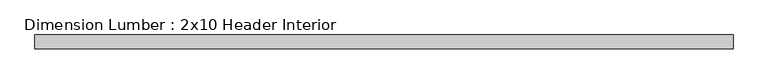
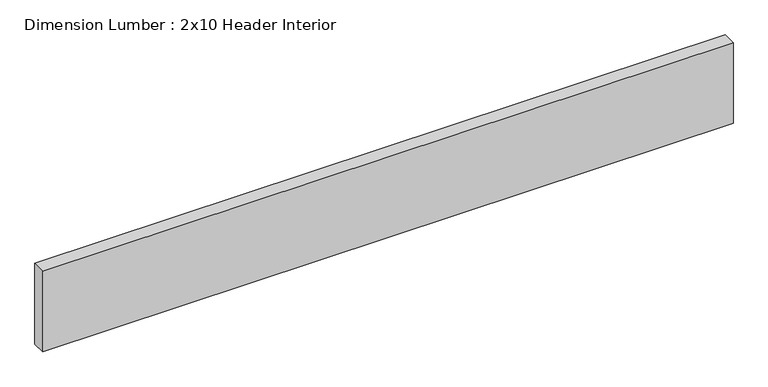
"""IFC4 building model written with IfcOpenShell, lengths in millimetres: beam geometry, Dimension Lumber : 2x10 Header Interior."""

import ifcopenshell
import ifcopenshell.guid

model = None  # the IFC model being written
_history = None  # IfcOwnerHistory: only IFC2X3 demands one
_inside = {}  # id of a spatial element -> (the spatial element, [elements in it])
_under = {}  # id of a project, library or spatial element -> (it, [spatial elements below it])
_declared = {}  # id of a project -> (the project, [libraries it declares])
_typed = {}  # id of a type object -> (the type object, [elements of that type])
_made_of = {}  # id of a material, layer set ... -> (it, [elements and type objects made of it])


def new_model(schema):
    """Start an empty IFC model of exactly this schema.

    Asked for "IFC4X3", IfcOpenShell would pick the latest addendum, in which some entities
    have other attributes; the version numbers below select the first issue.
    IFC2X3 requires an IfcOwnerHistory on every rooted entity: one is made here for all.
    """
    global model, _history
    if schema == "IFC4X3":
        model = ifcopenshell.file(schema_version=(4, 3, 0, 0))
    else:
        model = ifcopenshell.file(schema=schema)
    _inside.clear()
    _under.clear()
    _declared.clear()
    _typed.clear()
    _made_of.clear()
    _history = None
    if model.schema == "IFC2X3":
        org = make("IfcOrganization", Name="unknown")
        user = make(
            "IfcPersonAndOrganization",
            ThePerson=make("IfcPerson", FamilyName="unknown"),
            TheOrganization=org,
        )
        app = make(
            "IfcApplication",
            ApplicationDeveloper=org,
            Version="unknown",
            ApplicationFullName="unknown",
            ApplicationIdentifier="unknown",
        )
        _history = make(
            "IfcOwnerHistory",
            OwningUser=user,
            OwningApplication=app,
            ChangeAction="ADDED",
            CreationDate=0,
        )
    return model


def make(cls, **values):
    """One entity of the class cls with the attributes given. An attribute that is None is left unset."""
    return model.create_entity(
        cls, **{name: value for name, value in values.items() if value is not None}
    )


def rooted(cls, **values):
    """An entity with a GlobalId (a new one), such as an element, a storey or a relation."""
    return make(cls, GlobalId=ifcopenshell.guid.new(), OwnerHistory=_history, **values)


def si_unit(unit_type, name, prefix=None):
    """IfcSIUnit, for example si_unit("LENGTHUNIT", "METRE", prefix="MILLI")."""
    return make("IfcSIUnit", UnitType=unit_type, Prefix=prefix, Name=name)


def assignment(units):
    """IfcUnitAssignment: the units of a project."""
    return None if units is None else make("IfcUnitAssignment", Units=units)


def point(xyz):
    """IfcCartesianPoint."""
    return None if xyz is None else make("IfcCartesianPoint", Coordinates=xyz)


def direction(xyz):
    """IfcDirection."""
    return None if xyz is None else make("IfcDirection", DirectionRatios=xyz)


def frame(location, z_axis=None, x_axis=None):
    """IfcAxis2Placement3D, a coordinate frame: its origin and axes. An axis left out is left unset."""
    return make(
        "IfcAxis2Placement3D",
        Location=point(location),
        Axis=direction(z_axis),
        RefDirection=direction(x_axis),
    )


def origin():
    """The frame at (0, 0, 0) with its axes left unset."""
    return frame((0.0, 0.0, 0.0))


def place(relative_to, where):
    """IfcLocalPlacement: puts the frame where relative to a parent placement (None: the world)."""
    return make(
        "IfcLocalPlacement", PlacementRelTo=relative_to, RelativePlacement=where
    )


def context(
    kind, dimensions, precision=None, world=None, true_north=None, identifier=None
):
    """IfcGeometricRepresentationContext, for example the 3D "Model" context."""
    return make(
        "IfcGeometricRepresentationContext",
        ContextIdentifier=identifier,
        ContextType=kind,
        CoordinateSpaceDimension=dimensions,
        Precision=precision,
        WorldCoordinateSystem=world,
        TrueNorth=true_north,
    )


def project(units=None, contexts=None):
    """IfcProject with its units and contexts."""
    return rooted(
        "IfcProject",
        Name="project",
        RepresentationContexts=contexts,
        UnitsInContext=assignment(units),
    )


def spatial(cls, under=None, at=None, **own):
    """A site, building, storey or space (cls), placed at a placement, below another one or the project."""
    s = rooted(cls, ObjectPlacement=at, **own)
    if under is not None:
        _under.setdefault(under.id(), (under, []))[1].append(s)
    return s


def polyline(points):
    """IfcPolyline through the points."""
    return make("IfcPolyline", Points=[point(p) for p in points])


def outline(outer, holes=None, kind="AREA"):
    """IfcArbitraryClosedProfileDef: a profile drawn as a closed curve; with holes, ...WithVoids."""
    if holes is None:
        return make("IfcArbitraryClosedProfileDef", ProfileType=kind, OuterCurve=outer)
    return make(
        "IfcArbitraryProfileDefWithVoids",
        ProfileType=kind,
        OuterCurve=outer,
        InnerCurves=holes,
    )


def extrude(swept, where, along, depth):
    """IfcExtrudedAreaSolid: the profile swept, set in the frame where, extruded along a direction by depth."""
    return make(
        "IfcExtrudedAreaSolid",
        SweptArea=swept,
        Position=where,
        ExtrudedDirection=direction(along),
        Depth=depth,
    )


def shape(context_of_items, identifier, shape_type, items):
    """IfcShapeRepresentation: the items that make up one representation, for example the "Body"."""
    return make(
        "IfcShapeRepresentation",
        ContextOfItems=context_of_items,
        RepresentationIdentifier=identifier,
        RepresentationType=shape_type,
        Items=items,
    )


def source(mapping_origin, context_of_items, identifier, shape_type, items):
    """IfcRepresentationMap: a shape defined once, which mapped items show again and again."""
    return make(
        "IfcRepresentationMap",
        MappingOrigin=mapping_origin,
        MappedRepresentation=shape(context_of_items, identifier, shape_type, items),
    )


def transform(
    local_origin,
    x_axis=None,
    y_axis=None,
    z_axis=None,
    scale=None,
    scale2=None,
    scale3=None,
    uniform=True,
):
    """IfcCartesianTransformationOperator3D, or its non-uniform kind. x_axis, y_axis, z_axis: its Axis1, 2, 3."""
    if uniform:
        return make(
            "IfcCartesianTransformationOperator3D",
            Axis1=direction(x_axis),
            Axis2=direction(y_axis),
            LocalOrigin=point(local_origin),
            Scale=scale,
            Axis3=direction(z_axis),
        )
    return make(
        "IfcCartesianTransformationOperator3DnonUniform",
        Axis1=direction(x_axis),
        Axis2=direction(y_axis),
        LocalOrigin=point(local_origin),
        Scale=scale,
        Axis3=direction(z_axis),
        Scale2=scale2,
        Scale3=scale3,
    )


def mapped(mapping_source, mapping_target):
    """IfcMappedItem: shows the shape of a source again, moved by a transform."""
    return make(
        "IfcMappedItem", MappingSource=mapping_source, MappingTarget=mapping_target
    )


def made_of(thing, what):
    """Note that an element or type object is made of a material, layer set ...; save() writes the relation."""
    if what is not None:
        _made_of.setdefault(what.id(), (what, []))[1].append(thing)
    return thing


def element(
    cls,
    number,
    at=None,
    inside=None,
    cuts=None,
    type_object=None,
    material=None,
    context=None,
    identifier="Body",
    shape_type=None,
    held_by="IfcProductDefinitionShape",
    body=None,
    shapes=None,
    **own,
):
    """One element of the class cls, such as IfcWall. Its Tag is "e" and its number.

    at: its placement. inside: the storey or other place that contains it. cuts: it is an
    opening in that element (IfcRelVoidsElement). A single representation is given by context,
    identifier, shape_type and body (its items); several are given by shapes. held_by: the class
    of the entity that holds the representations. save() writes the other relations.
    """
    e = rooted(cls, Tag="e%d" % number, ObjectPlacement=at, **own)
    if body is not None:
        shapes = [shape(context, identifier, shape_type, body)]
    if shapes is not None:
        e.Representation = make(held_by, Representations=shapes)
    if inside is not None:
        _inside.setdefault(inside.id(), (inside, []))[1].append(e)
    if cuts is not None:
        rooted(
            "IfcRelVoidsElement", RelatingBuildingElement=cuts, RelatedOpeningElement=e
        )
    if type_object is not None:
        _typed.setdefault(type_object.id(), (type_object, []))[1].append(e)
    return made_of(e, material)


def aggregate(whole, parts):
    """IfcRelAggregates: a whole, such as a stair, and the parts it consists of."""
    return rooted("IfcRelAggregates", RelatingObject=whole, RelatedObjects=parts)


def save(model, path):
    """Write the relations noted so far, then the file.

    IfcRelAggregates (storeys below a building ...), IfcRelContainedInSpatialStructure (elements
    in a storey), IfcRelDefinesByType, IfcRelAssociatesMaterial and IfcRelDeclares: one each for
    every whole, place, type object, material and project.
    """
    for whole, parts in _under.values():
        aggregate(whole, parts)
    for where, things in _inside.values():
        rooted(
            "IfcRelContainedInSpatialStructure",
            RelatedElements=things,
            RelatingStructure=where,
        )
    for kind, things in _typed.values():
        rooted("IfcRelDefinesByType", RelatedObjects=things, RelatingType=kind)
    for what, things in _made_of.values():
        rooted("IfcRelAssociatesMaterial", RelatedObjects=things, RelatingMaterial=what)
    for by, libraries in _declared.values():
        rooted("IfcRelDeclares", RelatingContext=by, RelatedDefinitions=libraries)
    model.write(path)


def dimension_lumber_2x10_header_interior_91014728(model_context):
    return source(origin(), model_context, "Body", "SweptSolid", [
        extrude(outline(polyline([(468.709375, 19.05), (468.709375, -19.05), (-1434.7031244, -19.05), (-1434.7031244, 19.05), (468.709375, 19.05)])), frame((0.0, 0.0, -117.475), z_axis=(0.0, 0.0, 1.0), x_axis=(1.0, 0.0, 0.0)), (0.0, 0.0, 1.0), 234.95),
    ])


if __name__ == "__main__":
    model = new_model("IFC4")
    model_context = context("Model", 3, world=origin())
    ifc_project = project(units=[si_unit("LENGTHUNIT", "METRE", prefix="MILLI")], contexts=[model_context])
    site = spatial("IfcSite", under=ifc_project)
    building = spatial("IfcBuilding", under=site)
    placement = place(None, origin())
    dimension_lumber_2x10_header_interior_shape = dimension_lumber_2x10_header_interior_91014728(model_context)
    element("IfcBeam", 1, ObjectType="Dimension Lumber : 2x10 Header Interior", at=placement, inside=building, context=model_context, shape_type="MappedRepresentation", body=[
        mapped(dimension_lumber_2x10_header_interior_shape, transform((0.0, 0.0, 0.0), x_axis=(1.0, 0.0, 0.0), y_axis=(0.0, 1.0, 0.0), z_axis=(0.0, 0.0, 1.0))),
    ])
    save(model, "model.ifc")

# Revit data of these elements
# Type "Dimension Lumber : 2x10 Header Interior"
#   Assembly Code = "B10"
#   A = 0.0963889 SF
#   Length [instance default] = 5' - 0"
#   b = 0' - 1 1/2"
#   d = 0' - 9 1/4"
#   Structural Material [instance default] = Softwood, Lumber
# Element 1 (IfcBeam, "Dimension Lumber : 2x10 Header Interior")
#   Structural Material = Douglas Fir #2
#   Materials on its faces: "Douglas Fir #2"
# Materials
#   "Softwood, Lumber": class "Wood", colour RGB 223 192 134, transparency 0, Description = "Pinus Echinata", Cost = 0
#   "Douglas Fir #2": class "Wood", colour RGB 223 192 134, transparency 0, Description = "Pinus Echinata", Cost = 0
